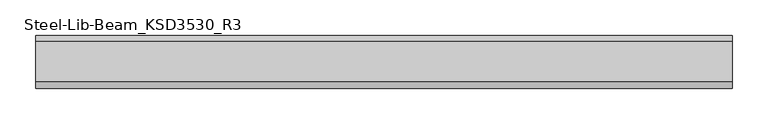
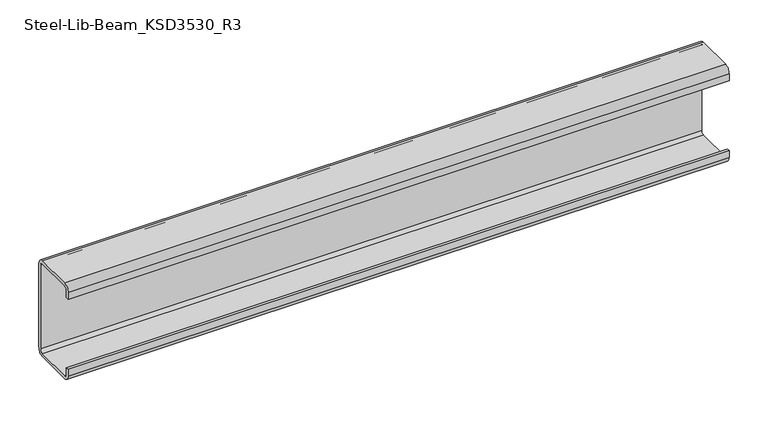
"""IFC4 building model written with IfcOpenShell, lengths in millimetres: beam geometry, Steel-Lib-Beam_KSD3530_R3 : BMS291_C-150×75x20x4.5."""

from ifc_helpers import new_model, si_unit, point, frame, frame_2d, origin, place, context, project, spatial, polyline, circle_curve, trimmed, segment, composite_curve, outline, extrude, source, transform, mapped, element, save


def steel_lib_beam_ksd3530_r3_533ee1bc(model_context):
    return source(origin(), model_context, "Body", "SweptSolid", [
        extrude(outline(composite_curve([segment(trimmed(circle_curve(frame_2d((-41.0, 66.0)), 9.0), [point((-50.0, 66.0))], [point((-41.0, 75.0))], False, "CARTESIAN"), True, "CONTINUOUS"), segment(polyline([(-41.0, 75.0), (16.0, 75.0)]), True, "CONTINUOUS"), segment(trimmed(circle_curve(frame_2d((16.0, 66.0)), 9.0), [point((16.0, 75.0))], [point((25.0, 66.0))], False, "CARTESIAN"), True, "CONTINUOUS"), segment(polyline([(25.0, 66.0), (25.0, -66.0)]), True, "CONTINUOUS"), segment(trimmed(circle_curve(frame_2d((16.0, -66.0)), 9.0), [point((25.0, -66.0))], [point((16.0, -75.0))], False, "CARTESIAN"), True, "CONTINUOUS"), segment(polyline([(16.0, -75.0), (-41.0, -75.0)]), True, "CONTINUOUS"), segment(trimmed(circle_curve(frame_2d((-41.0, -66.0)), 9.0), [point((-41.0, -75.0))], [point((-50.0, -66.0))], False, "CARTESIAN"), True, "CONTINUOUS"), segment(polyline([(-50.0, -66.0), (-50.0, -55.0), (-45.5, -55.0), (-45.5, -66.0)]), True, "CONTINUOUS"), segment(trimmed(circle_curve(frame_2d((-41.0, -66.0)), 4.5), [point((-45.5, -66.0))], [point((-41.0, -70.5))], True, "CARTESIAN"), True, "CONTINUOUS"), segment(polyline([(-41.0, -70.5), (16.0, -70.5)]), True, "CONTINUOUS"), segment(trimmed(circle_curve(frame_2d((16.0, -66.0)), 4.5), [point((16.0, -70.5))], [point((20.5, -66.0))], True, "CARTESIAN"), True, "CONTINUOUS"), segment(polyline([(20.5, -66.0), (20.5, 66.0)]), True, "CONTINUOUS"), segment(trimmed(circle_curve(frame_2d((16.0, 66.0)), 4.5), [point((20.5, 66.0))], [point((16.0, 70.5))], True, "CARTESIAN"), True, "CONTINUOUS"), segment(polyline([(16.0, 70.5), (-41.0, 70.5)]), True, "CONTINUOUS"), segment(trimmed(circle_curve(frame_2d((-41.0, 66.0)), 4.5), [point((-41.0, 70.5))], [point((-45.5, 66.0))], True, "CARTESIAN"), True, "CONTINUOUS"), segment(polyline([(-45.5, 66.0), (-45.5, 55.0), (-50.0, 55.0), (-50.0, 66.0)]), True, "CONTINUOUS")], self_intersect=False)), frame((-490.0, 0.0, 0.0), z_axis=(1.0, 0.0, 0.0), x_axis=(0.0, 1.0, 0.0)), (0.0, 0.0, 1.0), 980.0),
    ])


if __name__ == "__main__":
    model = new_model("IFC4")
    model_context = context("Model", 3, world=origin())
    ifc_project = project(units=[si_unit("LENGTHUNIT", "METRE", prefix="MILLI")], contexts=[model_context])
    site = spatial("IfcSite", under=ifc_project)
    building = spatial("IfcBuilding", under=site)
    placement = place(None, origin())
    steel_lib_beam_ksd3530_r3_shape = steel_lib_beam_ksd3530_r3_533ee1bc(model_context)
    element("IfcBeam", 1, ObjectType="Steel-Lib-Beam_KSD3530_R3 : BMS291_C-150×75x20x4.5", at=placement, inside=building, context=model_context, shape_type="MappedRepresentation", body=[
        mapped(steel_lib_beam_ksd3530_r3_shape, transform((0.0, 0.0, 0.0), x_axis=(1.0, 0.0, 0.0), y_axis=(0.0, 1.0, 0.0), z_axis=(0.0, 0.0, 1.0))),
    ])
    save(model, "model.ifc")

# Revit data of these elements
# Type "Steel-Lib-Beam_KSD3530_R3 : BMS291_C-150×75x20x4.5"
#   Keynote = "C-150×75x20x4.5"
#   SteelWeight = "Light"
#   x = 0.0250 m
#   t1 = 0.0090 m
#   t = 0.0045 m
#   Surface Area = 0.629834 m²/m
#   Section Area = 13.9688 cm²
#   Mass per Unit Length = 10.9655 kg/m
#   C = 0.0200 m
#   A = 0.0750 m
#   Length [instance default] = 1.5000 m
#   H = 0.1500 m
#   hec_material4 [instance default] = none
#   hec_material3 [instance default] = none
#   hec_material2 [instance default] = none
#   hec_material1 [instance default] = none
#   Structural Material [instance default] = Metal - Steel - Light Gauge
#   Assembly Code = ""
# Element 1 (IfcBeam, "Steel-Lib-Beam_KSD3530_R3 : BMS291_C-150×75x20x4.5")
#   Structural Material = none
# Materials
#   "Metal - Steel - Light Gauge": class "Metal", colour RGB 247 247 247, transparency 0
